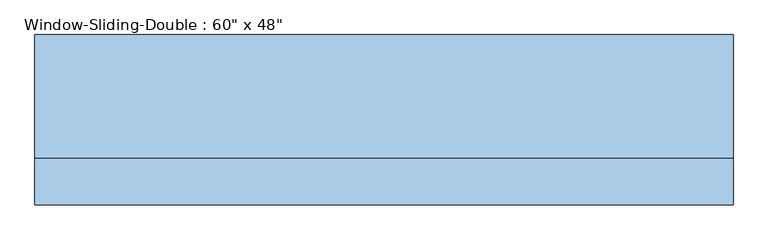
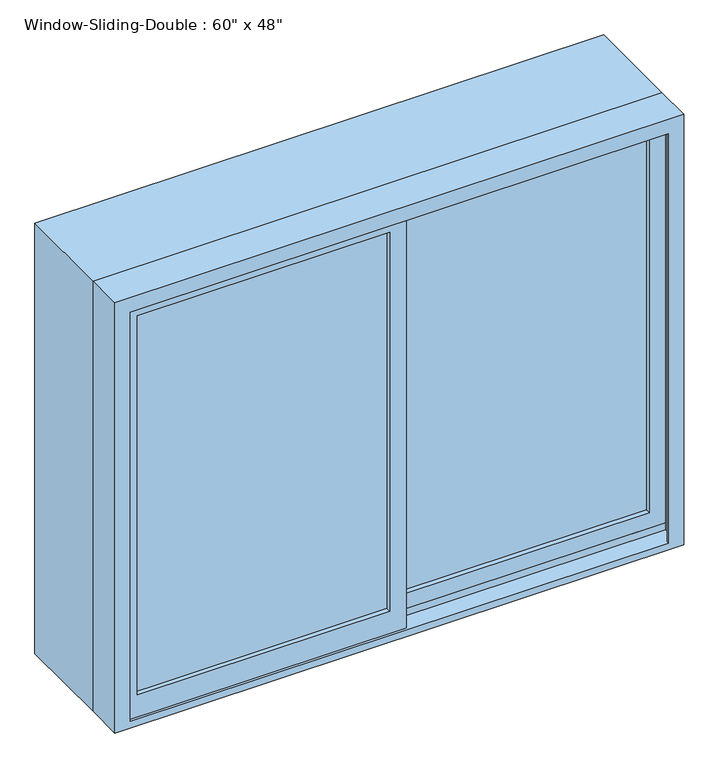
"""IFC4 building model written with IfcOpenShell, lengths in millimetres: window geometry."""

import ifcopenshell
import ifcopenshell.guid

model = None  # the IFC model being written
_history = None  # IfcOwnerHistory: only IFC2X3 demands one
_inside = {}  # id of a spatial element -> (the spatial element, [elements in it])
_under = {}  # id of a project, library or spatial element -> (it, [spatial elements below it])
_declared = {}  # id of a project -> (the project, [libraries it declares])
_typed = {}  # id of a type object -> (the type object, [elements of that type])
_made_of = {}  # id of a material, layer set ... -> (it, [elements and type objects made of it])


def new_model(schema):
    """Start an empty IFC model of exactly this schema.

    Asked for "IFC4X3", IfcOpenShell would pick the latest addendum, in which some entities
    have other attributes; the version numbers below select the first issue.
    IFC2X3 requires an IfcOwnerHistory on every rooted entity: one is made here for all.
    """
    global model, _history
    if schema == "IFC4X3":
        model = ifcopenshell.file(schema_version=(4, 3, 0, 0))
    else:
        model = ifcopenshell.file(schema=schema)
    _inside.clear()
    _under.clear()
    _declared.clear()
    _typed.clear()
    _made_of.clear()
    _history = None
    if model.schema == "IFC2X3":
        org = make("IfcOrganization", Name="unknown")
        user = make(
            "IfcPersonAndOrganization",
            ThePerson=make("IfcPerson", FamilyName="unknown"),
            TheOrganization=org,
        )
        app = make(
            "IfcApplication",
            ApplicationDeveloper=org,
            Version="unknown",
            ApplicationFullName="unknown",
            ApplicationIdentifier="unknown",
        )
        _history = make(
            "IfcOwnerHistory",
            OwningUser=user,
            OwningApplication=app,
            ChangeAction="ADDED",
            CreationDate=0,
        )
    return model


def make(cls, **values):
    """One entity of the class cls with the attributes given. An attribute that is None is left unset."""
    return model.create_entity(
        cls, **{name: value for name, value in values.items() if value is not None}
    )


def rooted(cls, **values):
    """An entity with a GlobalId (a new one), such as an element, a storey or a relation."""
    return make(cls, GlobalId=ifcopenshell.guid.new(), OwnerHistory=_history, **values)


def si_unit(unit_type, name, prefix=None):
    """IfcSIUnit, for example si_unit("LENGTHUNIT", "METRE", prefix="MILLI")."""
    return make("IfcSIUnit", UnitType=unit_type, Prefix=prefix, Name=name)


def assignment(units):
    """IfcUnitAssignment: the units of a project."""
    return None if units is None else make("IfcUnitAssignment", Units=units)


def point(xyz):
    """IfcCartesianPoint."""
    return None if xyz is None else make("IfcCartesianPoint", Coordinates=xyz)


def direction(xyz):
    """IfcDirection."""
    return None if xyz is None else make("IfcDirection", DirectionRatios=xyz)


def frame(location, z_axis=None, x_axis=None):
    """IfcAxis2Placement3D, a coordinate frame: its origin and axes. An axis left out is left unset."""
    return make(
        "IfcAxis2Placement3D",
        Location=point(location),
        Axis=direction(z_axis),
        RefDirection=direction(x_axis),
    )


def origin():
    """The frame at (0, 0, 0) with its axes left unset."""
    return frame((0.0, 0.0, 0.0))


def place(relative_to, where):
    """IfcLocalPlacement: puts the frame where relative to a parent placement (None: the world)."""
    return make(
        "IfcLocalPlacement", PlacementRelTo=relative_to, RelativePlacement=where
    )


def context(
    kind, dimensions, precision=None, world=None, true_north=None, identifier=None
):
    """IfcGeometricRepresentationContext, for example the 3D "Model" context."""
    return make(
        "IfcGeometricRepresentationContext",
        ContextIdentifier=identifier,
        ContextType=kind,
        CoordinateSpaceDimension=dimensions,
        Precision=precision,
        WorldCoordinateSystem=world,
        TrueNorth=true_north,
    )


def project(units=None, contexts=None):
    """IfcProject with its units and contexts."""
    return rooted(
        "IfcProject",
        Name="project",
        RepresentationContexts=contexts,
        UnitsInContext=assignment(units),
    )


def spatial(cls, under=None, at=None, **own):
    """A site, building, storey or space (cls), placed at a placement, below another one or the project."""
    s = rooted(cls, ObjectPlacement=at, **own)
    if under is not None:
        _under.setdefault(under.id(), (under, []))[1].append(s)
    return s


def polyline(points):
    """IfcPolyline through the points."""
    return make("IfcPolyline", Points=[point(p) for p in points])


def outline(outer, holes=None, kind="AREA"):
    """IfcArbitraryClosedProfileDef: a profile drawn as a closed curve; with holes, ...WithVoids."""
    if holes is None:
        return make("IfcArbitraryClosedProfileDef", ProfileType=kind, OuterCurve=outer)
    return make(
        "IfcArbitraryProfileDefWithVoids",
        ProfileType=kind,
        OuterCurve=outer,
        InnerCurves=holes,
    )


def extrude(swept, where, along, depth):
    """IfcExtrudedAreaSolid: the profile swept, set in the frame where, extruded along a direction by depth."""
    return make(
        "IfcExtrudedAreaSolid",
        SweptArea=swept,
        Position=where,
        ExtrudedDirection=direction(along),
        Depth=depth,
    )


def faces_of(points, faces, orient=None, outer=None):
    """IfcFace entities. A face is a list of loops; a loop is a list of indices into points, from 0.

    orient and outer hold one flag for each loop. By default every Orientation is true, the
    first loop of a face is its IfcFaceOuterBound and the others are IfcFaceBound.
    """
    made = []
    for i, loops in enumerate(faces):
        bounds = []
        for j, loop in enumerate(loops):
            is_outer = j == 0 if outer is None else outer[i][j]
            bounds.append(
                make(
                    "IfcFaceOuterBound" if is_outer else "IfcFaceBound",
                    Bound=make("IfcPolyLoop", Polygon=[points[k] for k in loop]),
                    Orientation=True if orient is None else orient[i][j],
                )
            )
        made.append(make("IfcFace", Bounds=bounds))
    return made


def faceted_brep(points, faces, orient=None, outer=None, voids=None):
    """IfcFacetedBrep: a solid bounded by flat faces; with voids (closed shells), ...WithVoids."""
    shared = [point(p) for p in points]
    hull = make("IfcClosedShell", CfsFaces=faces_of(shared, faces, orient, outer))
    if voids is None:
        return make("IfcFacetedBrep", Outer=hull)
    return make(
        "IfcFacetedBrepWithVoids",
        Outer=hull,
        Voids=[
            make(cls, CfsFaces=faces_of(shared, fs, o, b)) for cls, fs, o, b in voids
        ],
    )


def shape(context_of_items, identifier, shape_type, items):
    """IfcShapeRepresentation: the items that make up one representation, for example the "Body"."""
    return make(
        "IfcShapeRepresentation",
        ContextOfItems=context_of_items,
        RepresentationIdentifier=identifier,
        RepresentationType=shape_type,
        Items=items,
    )


def source(mapping_origin, context_of_items, identifier, shape_type, items):
    """IfcRepresentationMap: a shape defined once, which mapped items show again and again."""
    return make(
        "IfcRepresentationMap",
        MappingOrigin=mapping_origin,
        MappedRepresentation=shape(context_of_items, identifier, shape_type, items),
    )


def transform(
    local_origin,
    x_axis=None,
    y_axis=None,
    z_axis=None,
    scale=None,
    scale2=None,
    scale3=None,
    uniform=True,
):
    """IfcCartesianTransformationOperator3D, or its non-uniform kind. x_axis, y_axis, z_axis: its Axis1, 2, 3."""
    if uniform:
        return make(
            "IfcCartesianTransformationOperator3D",
            Axis1=direction(x_axis),
            Axis2=direction(y_axis),
            LocalOrigin=point(local_origin),
            Scale=scale,
            Axis3=direction(z_axis),
        )
    return make(
        "IfcCartesianTransformationOperator3DnonUniform",
        Axis1=direction(x_axis),
        Axis2=direction(y_axis),
        LocalOrigin=point(local_origin),
        Scale=scale,
        Axis3=direction(z_axis),
        Scale2=scale2,
        Scale3=scale3,
    )


def mapped(mapping_source, mapping_target):
    """IfcMappedItem: shows the shape of a source again, moved by a transform."""
    return make(
        "IfcMappedItem", MappingSource=mapping_source, MappingTarget=mapping_target
    )


def made_of(thing, what):
    """Note that an element or type object is made of a material, layer set ...; save() writes the relation."""
    if what is not None:
        _made_of.setdefault(what.id(), (what, []))[1].append(thing)
    return thing


def element(
    cls,
    number,
    at=None,
    inside=None,
    cuts=None,
    type_object=None,
    material=None,
    context=None,
    identifier="Body",
    shape_type=None,
    held_by="IfcProductDefinitionShape",
    body=None,
    shapes=None,
    **own,
):
    """One element of the class cls, such as IfcWall. Its Tag is "e" and its number.

    at: its placement. inside: the storey or other place that contains it. cuts: it is an
    opening in that element (IfcRelVoidsElement). A single representation is given by context,
    identifier, shape_type and body (its items); several are given by shapes. held_by: the class
    of the entity that holds the representations. save() writes the other relations.
    """
    e = rooted(cls, Tag="e%d" % number, ObjectPlacement=at, **own)
    if body is not None:
        shapes = [shape(context, identifier, shape_type, body)]
    if shapes is not None:
        e.Representation = make(held_by, Representations=shapes)
    if inside is not None:
        _inside.setdefault(inside.id(), (inside, []))[1].append(e)
    if cuts is not None:
        rooted(
            "IfcRelVoidsElement", RelatingBuildingElement=cuts, RelatedOpeningElement=e
        )
    if type_object is not None:
        _typed.setdefault(type_object.id(), (type_object, []))[1].append(e)
    return made_of(e, material)


def aggregate(whole, parts):
    """IfcRelAggregates: a whole, such as a stair, and the parts it consists of."""
    return rooted("IfcRelAggregates", RelatingObject=whole, RelatedObjects=parts)


def save(model, path):
    """Write the relations noted so far, then the file.

    IfcRelAggregates (storeys below a building ...), IfcRelContainedInSpatialStructure (elements
    in a storey), IfcRelDefinesByType, IfcRelAssociatesMaterial and IfcRelDeclares: one each for
    every whole, place, type object, material and project.
    """
    for whole, parts in _under.values():
        aggregate(whole, parts)
    for where, things in _inside.values():
        rooted(
            "IfcRelContainedInSpatialStructure",
            RelatedElements=things,
            RelatingStructure=where,
        )
    for kind, things in _typed.values():
        rooted("IfcRelDefinesByType", RelatedObjects=things, RelatingType=kind)
    for what, things in _made_of.values():
        rooted("IfcRelAssociatesMaterial", RelatedObjects=things, RelatingMaterial=what)
    for by, libraries in _declared.values():
        rooted("IfcRelDeclares", RelatingContext=by, RelatedDefinitions=libraries)
    model.write(path)


def window_a5531389(model_context):
    return source(origin(), model_context, "Body", "SolidModel", [
        faceted_brep([(-762.0, -89.8525, 914.4), (762.0, -89.8525, 914.4), (762.0, -191.4525, 914.4), (-762.0, -191.4525, 914.4), (-721.0778905, -191.4525, 2092.6778905), (-721.0778905, -191.4525, 933.45), (-721.0778905, -185.1025, 933.45), (-721.0778905, -185.1025, 2092.6778905), (-742.95, -185.1025, 933.45), (-742.95, -185.1025, 2114.55), (742.95, -185.1025, 2114.55), (742.95, -185.1025, 933.45), (721.0778905, -185.1025, 933.45), (721.0778905, -185.1025, 2092.6778905), (-742.95, -140.6525, 933.45), (-742.95, -140.6525, 952.5), (-742.95, -96.2025, 952.5), (-742.95, -96.2025, 933.45), (-742.95, -89.8525, 933.45), (-742.95, -89.8525, 2114.55), (-762.0, -89.8525, 2133.6), (762.0, -89.8525, 2133.6), (742.95, -89.8525, 2114.55), (742.95, -89.8525, 933.45), (-762.0, -191.4525, 2133.6), (762.0, -191.4525, 2133.6), (721.0778905, -191.4525, 2092.6778905), (721.0778905, -191.4525, 933.45), (742.95, -96.2025, 933.45), (742.95, -96.2025, 952.5), (742.95, -140.6525, 952.5), (742.95, -140.6525, 933.45)], [[[0, 1, 2, 3]], [[4, 5, 6, 7]], [[7, 6, 8, 9, 10, 11, 12, 13]], [[9, 8, 14, 15, 16, 17, 18, 19]], [[0, 20, 21, 1], [22, 19, 18, 23]], [[24, 20, 0, 3]], [[2, 25, 24, 3], [4, 26, 27, 5]], [[7, 13, 26, 4]], [[9, 19, 22, 10]], [[20, 24, 25, 21]], [[13, 12, 27, 26]], [[22, 23, 28, 29, 30, 31, 11, 10]], [[21, 25, 2, 1]], [[27, 12, 11, 31, 14, 8, 6, 5]], [[31, 30, 15, 14]], [[30, 29, 16, 15]], [[29, 28, 17, 16]], [[18, 17, 28, 23]]]),
        extrude(outline(polyline([(2133.6, 762.0), (2133.6, -762.0), (914.4, -762.0), (914.4, 762.0), (2133.6, 762.0)]), holes=[polyline([(2114.55, -742.95), (2114.55, 742.95), (933.45, 742.95), (933.45, -742.95), (2114.55, -742.95)])]), frame((0.0, -89.8525, 0.0), z_axis=(0.0, 1.0, 0.0), x_axis=(0.0, 0.0, 1.0)), (0.0, 0.0, 1.0), 269.875),
        extrude(outline(polyline([(698.5, -127.9525), (22.225, -127.9525), (22.225, -121.6025), (698.5, -121.6025), (698.5, -127.9525)])), frame((0.0, 0.0, 996.95), z_axis=(0.0, 0.0, 1.0), x_axis=(1.0, 0.0, 0.0)), (0.0, 0.0, 1.0), 1073.15),
        extrude(outline(polyline([(698.5, -115.2525), (22.225, -115.2525), (22.225, -108.9025), (698.5, -108.9025), (698.5, -115.2525)])), frame((0.0, 0.0, 996.95), z_axis=(0.0, 0.0, 1.0), x_axis=(1.0, 0.0, 0.0)), (0.0, 0.0, 1.0), 1073.15),
        extrude(outline(polyline([(-22.225, -172.4025), (-698.5, -172.4025), (-698.5, -166.0525), (-22.225, -166.0525), (-22.225, -172.4025)])), frame((0.0, 0.0, 996.95), z_axis=(0.0, 0.0, 1.0), x_axis=(1.0, 0.0, 0.0)), (0.0, 0.0, 1.0), 1073.15),
        extrude(outline(polyline([(-22.225, -159.7025), (-698.5, -159.7025), (-698.5, -153.3525), (-22.225, -153.3525), (-22.225, -159.7025)])), frame((0.0, 0.0, 996.95), z_axis=(0.0, 0.0, 1.0), x_axis=(1.0, 0.0, 0.0)), (0.0, 0.0, 1.0), 1073.15),
        extrude(outline(polyline([(933.45, 22.225), (2114.55, 22.225), (2114.55, -742.95), (933.45, -742.95), (933.45, 22.225)]), holes=[polyline([(2070.1, -698.5), (2070.1, -22.225), (996.95, -22.225), (996.95, -698.5), (2070.1, -698.5)])]), frame((0.0, -185.1025, 0.0), z_axis=(0.0, 1.0, 0.0), x_axis=(0.0, 0.0, 1.0)), (0.0, 0.0, 1.0), 44.45),
        extrude(outline(polyline([(952.5, -22.225), (952.5, 742.95), (2114.55, 742.95), (2114.55, -22.225), (952.5, -22.225)]), holes=[polyline([(996.95, 698.5), (996.95, 22.225), (2070.1, 22.225), (2070.1, 698.5), (996.95, 698.5)])]), frame((0.0, -140.6525, 0.0), z_axis=(0.0, 1.0, 0.0), x_axis=(0.0, 0.0, 1.0)), (0.0, 0.0, 1.0), 44.45),
    ])


if __name__ == "__main__":
    model = new_model("IFC4")
    model_context = context("Model", 3, world=origin())
    ifc_project = project(units=[si_unit("LENGTHUNIT", "METRE", prefix="MILLI")], contexts=[model_context])
    site = spatial("IfcSite", under=ifc_project)
    building = spatial("IfcBuilding", under=site)
    placement = place(None, origin())
    window_shape = window_a5531389(model_context)
    element("IfcWindow", 1, ObjectType="Window-Sliding-Double : 60\" x 48\"", at=placement, inside=building, context=model_context, shape_type="MappedRepresentation", body=[
        mapped(window_shape, transform((0.0, 0.0, 0.0), x_axis=(1.0, 0.0, 0.0), y_axis=(0.0, 1.0, 0.0), z_axis=(0.0, 0.0, 1.0))),
    ])
    save(model, "model.ifc")

# Revit data of these elements
# Type "Window-Sliding-Double : 60\" x 48\""
#   Type Mark = "13"
#   Fire Rating = "0.5h"
#   Assembly Code = "B2020100"
#   Analytic Construction = "Double glazing - domestic"
#   Window Inset [instance default] = 0' - 0"
#   Wall Thickness [instance default] = 0' - 6"
#   Visual Light Transmittance = 0.81
#   Thermal Resistance (R) = 1.8146 (h·ft²·°F)/BTU
#   Solar Heat Gain Coefficient = 0.76
#   Muntin Width = 2' - 2 5/8"
#   Muntin Height = 3' - 6 1/4"
#   Interior Wall Closure [instance default] = 0' - 2 3/4"
#   Heat Transfer Coefficient (U) = 0.5511 BTU/(h·ft²·°F)
#   Frame Extension [instance default] = 0' - 0 1/4"
#   Exterior Wall Closure [instance default] = 0' - 1 1/4"
#   Rough Width = 5' - 0 1/2"
#   Rough Height = 4' - 0 1/2"
#   Height = 4' - 0"
#   Extension Jamb [instance default] = 0' - 2 3/4"
#   Default Sill Height = 3' - 0"
#   Width = 5' - 0"
#   Interior Trim Visibility [instance default] = yes
#   Indicator Visibility [instance default] = yes
#   Exterior Trim Visibility [instance default] = yes
#   Muntin Visibility = yes
#   Extension Jamb Visibility [instance default] = yes
#   Define Thermal Properties by = 1
#   Muntin Pattern = Muntin Pattern_2x2 : Muntin Pattern_2x2
#   Interior Trim Material = Cherry
#   Interior Trim = Trim-Window-Interior-Flat : Picture Frame
#   Interior Frame Material = Cherry
#   Glass Panel Material = Glass, Clear Glazing
#   Exterior Trim Material = PVC, Flexible
#   Exterior Trim = Trim-Window-Exterior-Flat : with Sill
#   Exterior Frame Material = PVC, Flexible
#   Wall Closure = (empty or 0)
# Element 1 (IfcWindow, "Window-Sliding-Double : 60\" x 48\"")
#   Wall Thickness = 1' - 1 7/8"
#   Extension Jamb = 0' - 10 5/8"
#   Materials on its faces: "Cherry", "Glass, Clear Glazing", "PVC, Flexible"
# Materials
#   "Cherry": class "Wood", colour RGB 157 77 38, transparency 0, Description = "Prunus Serotina", Cost = 0
#   "Glass, Clear Glazing": class "Glass", colour RGB 120 120 120, transparency 0, Description = "Clear glazing", Cost = 0
#   "PVC, Flexible": class "Plastic", colour RGB 178 178 178, transparency 0, Description = "Flexible polyvinyl chloride", Cost = 0
